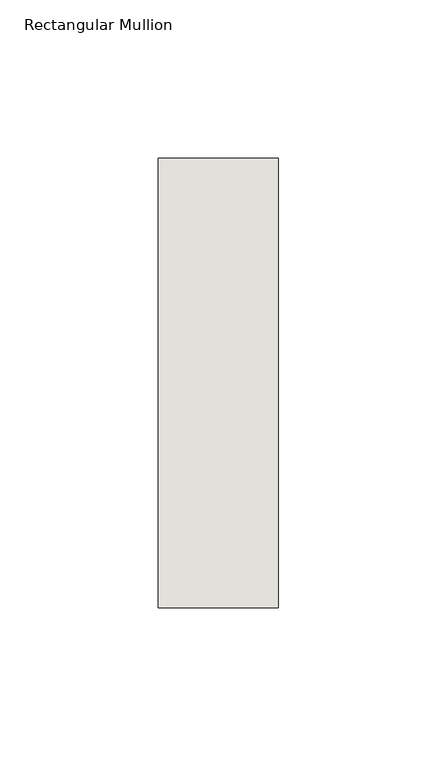
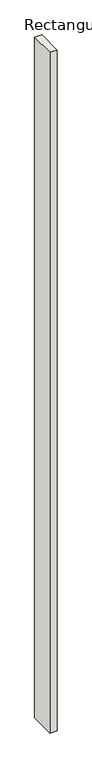
"""IFC4 building model written with IfcOpenShell, lengths in millimetres: wall geometry, Rectangular Mullion : NLRS_21_CWM_hsb-regel 38x142_gen_rsf."""

from ifc_helpers import new_model, si_unit, frame, origin, place, context, project, spatial, polyline, outline, extrude, source, transform, mapped, element, save


def rectangular_mullion_bc699282(model_context):
    return source(origin(), model_context, "Body", "SweptSolid", [
        extrude(outline(polyline([(19.0, -71.0), (-19.0, -71.0), (-19.0, 71.0), (19.0, 71.0), (19.0, -71.0)])), frame((0.0, 0.0, -3849.0), z_axis=(0.0, 0.0, 1.0), x_axis=(1.0, 0.0, 0.0)), (0.0, 0.0, 1.0), 3849.0),
    ])


if __name__ == "__main__":
    model = new_model("IFC4")
    model_context = context("Model", 3, world=origin())
    ifc_project = project(units=[si_unit("LENGTHUNIT", "METRE", prefix="MILLI")], contexts=[model_context])
    site = spatial("IfcSite", under=ifc_project)
    building = spatial("IfcBuilding", under=site)
    placement = place(None, origin())
    rectangular_mullion_shape = rectangular_mullion_bc699282(model_context)
    element("IfcWall", 1, ObjectType="Rectangular Mullion : NLRS_21_CWM_hsb-regel 38x142_gen_rsf", at=placement, inside=building, context=model_context, shape_type="MappedRepresentation", body=[
        mapped(rectangular_mullion_shape, transform((0.0, 0.0, 0.0), x_axis=(1.0, 0.0, 0.0), y_axis=(0.0, 1.0, 0.0), z_axis=(0.0, 0.0, 1.0))),
    ])
    save(model, "model.ifc")

# Revit data of these elements
# Type "Rectangular Mullion : NLRS_21_CWM_hsb-regel 38x142_gen_rsf"
#   Type IfcGUID = "07M7mRoiH1CR8m_RSKIwpF"
#   Assembly Code = "21.10"
#   IfcExportAs = "IfcWall"
#   built-in parameter 1007322 = 0.465879 (stored number, unit not read)
#   built-in parameter 1007321 = 0.062336 (stored number, unit not read)
#   built-in parameter 1007320 = 0.062336 (stored number, unit not read)
# Element 1 (IfcWall, "Rectangular Mullion : NLRS_21_CWM_hsb-regel 38x142_gen_rsf")
#   Materials on its faces: "NLRS_i2_hout naaldhout vuren_gen_rsf"
# Materials
#   "NLRS_i2_hout naaldhout vuren_gen_rsf": class "I - Hout", colour RGB 234 199 147, transparency 0, Keynote = "i2", Manufacturer = "Revit Standards Foundation", URL = "www.revitstandards.org", Description = "hout vuren", Cost = 0
